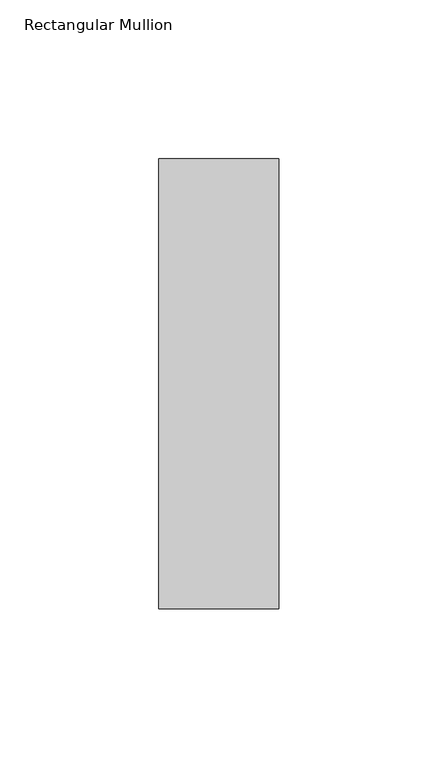
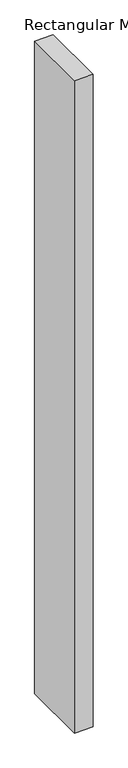
"""IFC4 building model written with IfcOpenShell, lengths in millimetres: member geometry, Rectangular Mullion : NLRS_21_CWM_hsb-regel 38x142_gen_rsf."""

from ifc_helpers import new_model, si_unit, frame, origin, place, context, project, spatial, polyline, outline, extrude, source, transform, mapped, element, save


def rectangular_mullion_d24150c1(model_context):
    return source(origin(), model_context, "Body", "SweptSolid", [
        extrude(outline(polyline([(19.0, -71.0), (-19.0, -71.0), (-19.0, 71.0), (19.0, 71.0), (19.0, -71.0)])), frame((0.0, 0.0, -1421.0), z_axis=(0.0, 0.0, 1.0), x_axis=(1.0, 0.0, 0.0)), (0.0, 0.0, 1.0), 1421.0),
    ])


if __name__ == "__main__":
    model = new_model("IFC4")
    model_context = context("Model", 3, world=origin())
    ifc_project = project(units=[si_unit("LENGTHUNIT", "METRE", prefix="MILLI")], contexts=[model_context])
    site = spatial("IfcSite", under=ifc_project)
    building = spatial("IfcBuilding", under=site)
    placement = place(None, origin())
    rectangular_mullion_shape = rectangular_mullion_d24150c1(model_context)
    element("IfcMember", 1, ObjectType="Rectangular Mullion : NLRS_21_CWM_hsb-regel 38x142_gen_rsf", at=placement, inside=building, context=model_context, shape_type="MappedRepresentation", body=[
        mapped(rectangular_mullion_shape, transform((0.0, 0.0, 0.0), x_axis=(1.0, 0.0, 0.0), y_axis=(0.0, 1.0, 0.0), z_axis=(0.0, 0.0, 1.0))),
    ])
    save(model, "model.ifc")

# Revit data of these elements
# Type "Rectangular Mullion : NLRS_21_CWM_hsb-regel 38x142_gen_rsf"
#   Export Type to IFC As = "IfcWall"
#   Type IfcGUID = "07M7mRoiH1CR8m_RSKIwpF"
#   Assembly Code = "21.10"
#   built-in parameter 1007322 = 0.465879 (stored number, unit not read)
#   built-in parameter 1007321 = 0.062336 (stored number, unit not read)
#   built-in parameter 1007320 = 0.062336 (stored number, unit not read)
# Element 1 (IfcMember, "Rectangular Mullion : NLRS_21_CWM_hsb-regel 38x142_gen_rsf")
#   Materials on its faces: "NLRS_i2_hout naaldhout vuren_gen_rsf"
# Materials
#   "NLRS_i2_hout naaldhout vuren_gen_rsf": class "I - Hout", colour RGB 234 199 147, transparency 0, Keynote = "i2", Manufacturer = "Revit Standards Foundation", URL = "www.revitstandards.org", Description = "hout vuren", Cost = 0
